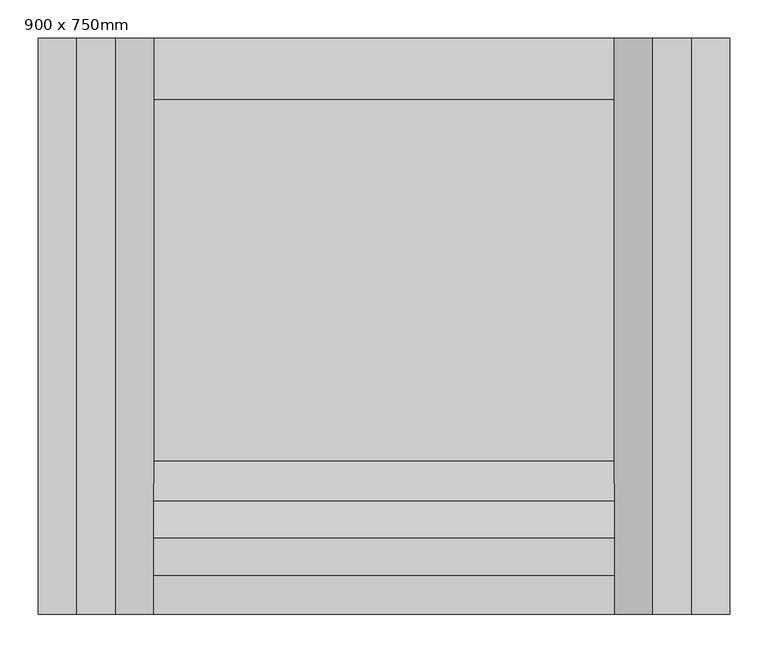
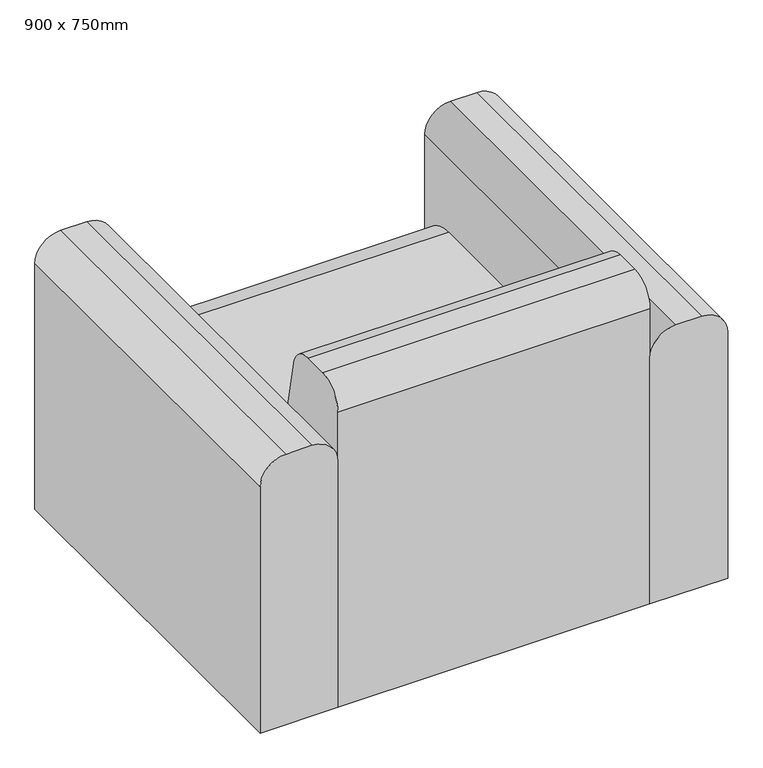
"""IFC4 building model written with IfcOpenShell, lengths in millimetres: furniture geometry, ソファ－I型 : 900 x 750mm."""

from ifc_helpers import new_model, si_unit, point, frame, frame_2d, origin, place, context, project, spatial, polyline, circle_curve, trimmed, segment, composite_curve, outline, extrude, source, transform, mapped, element, save


def furniture_900_x_750mm_fd91caf9(model_context):
    return source(origin(), model_context, "Body", "SweptSolid", [
        extrude(outline(composite_curve([segment(trimmed(circle_curve(frame_2d((500.0, -400.0)), 50.0), [point((550.0, -400.0))], [point((500.0, -450.0))], False, "CARTESIAN"), True, "CONTINUOUS"), segment(polyline([(500.0, -450.0), (0.0, -450.0), (0.0, -300.0), (500.0, -300.0)]), True, "CONTINUOUS"), segment(trimmed(circle_curve(frame_2d((500.0, -350.0)), 50.0), [point((500.0, -300.0))], [point((550.0, -350.0))], False, "CARTESIAN"), True, "CONTINUOUS"), segment(polyline([(550.0, -350.0), (550.0, -400.0)]), True, "CONTINUOUS")], self_intersect=False)), frame((0.0, -375.0, 0.0), z_axis=(0.0, 1.0, 0.0), x_axis=(0.0, 0.0, 1.0)), (0.0, 0.0, 1.0), 750.0),
        extrude(outline(composite_curve([segment(polyline([(550.0, 400.0), (550.0, 350.0)]), True, "CONTINUOUS"), segment(trimmed(circle_curve(frame_2d((500.0, 350.0)), 50.0), [point((550.0, 350.0))], [point((500.0, 300.0))], False, "CARTESIAN"), True, "CONTINUOUS"), segment(polyline([(500.0, 300.0), (0.0, 300.0), (0.0, 450.0), (500.0, 450.0)]), True, "CONTINUOUS"), segment(trimmed(circle_curve(frame_2d((500.0, 400.0)), 50.0), [point((500.0, 450.0))], [point((550.0, 400.0))], False, "CARTESIAN"), True, "CONTINUOUS")], self_intersect=False)), frame((0.0, -375.0, 0.0), z_axis=(0.0, 1.0, 0.0), x_axis=(0.0, 0.0, 1.0)), (0.0, 0.0, 1.0), 750.0),
        extrude(outline(composite_curve([segment(polyline([(-226.9611614, 609.8058068), (-175.0, 350.0), (295.0, 350.0)]), True, "CONTINUOUS"), segment(trimmed(circle_curve(frame_2d((295.0, 270.0)), 80.0), [point((295.0, 350.0))], [point((375.0, 270.0))], False, "CARTESIAN"), True, "CONTINUOUS"), segment(polyline([(375.0, 270.0), (375.0, 60.0), (305.0, 60.0), (305.0, 0.0), (-375.0, 0.0), (-375.0, 600.0)]), True, "CONTINUOUS"), segment(trimmed(circle_curve(frame_2d((-325.0, 600.0)), 50.0), [point((-375.0, 600.0))], [point((-325.0, 650.0))], False, "CARTESIAN"), True, "CONTINUOUS"), segment(polyline([(-325.0, 650.0), (-275.9901951, 650.0)]), True, "CONTINUOUS"), segment(trimmed(circle_curve(frame_2d((-275.9901951, 600.0)), 50.0), [point((-275.9901951, 650.0))], [point((-226.9611614, 609.8058068))], False, "CARTESIAN"), True, "CONTINUOUS")], self_intersect=False)), frame((-300.0, 0.0, 0.0), z_axis=(1.0, 0.0, 0.0), x_axis=(0.0, 1.0, 0.0)), (0.0, 0.0, 1.0), 600.0),
    ])


if __name__ == "__main__":
    model = new_model("IFC4")
    model_context = context("Model", 3, world=origin())
    ifc_project = project(units=[si_unit("LENGTHUNIT", "METRE", prefix="MILLI")], contexts=[model_context])
    site = spatial("IfcSite", under=ifc_project)
    building = spatial("IfcBuilding", under=site)
    placement = place(None, origin())
    furniture_900_x_750mm_shape = furniture_900_x_750mm_fd91caf9(model_context)
    element("IfcFurniture", 1, ObjectType="ソファ－I型 : 900 x 750mm", at=placement, inside=building, context=model_context, shape_type="MappedRepresentation", body=[
        mapped(furniture_900_x_750mm_shape, transform((0.0, 0.0, 0.0), x_axis=(1.0, 0.0, 0.0), y_axis=(0.0, 1.0, 0.0), z_axis=(0.0, 0.0, 1.0))),
    ])
    save(model, "model.ifc")

# Revit data of these elements
# Type "ソファ－I型 : 900 x 750mm"
#   Keynote = "12490.Y1"
#   座面高さ = 350 mm
#   幅 = 900 mm
#   奥行き = 750 mm
#   本体 = モチアミ - 無地 - グレー
#   Default Elevation = 0
# Element 1 (IfcFurniture, "ソファ－I型 : 900 x 750mm")
#   Materials on its faces: "モチアミ - 無地 - グレー"
# Materials
#   "モチアミ - 無地 - グレー": class "モチアミ", colour RGB 65 63 65, transparency 0, Cost = 0
